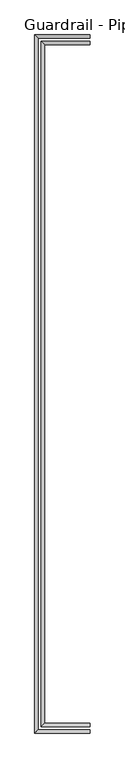
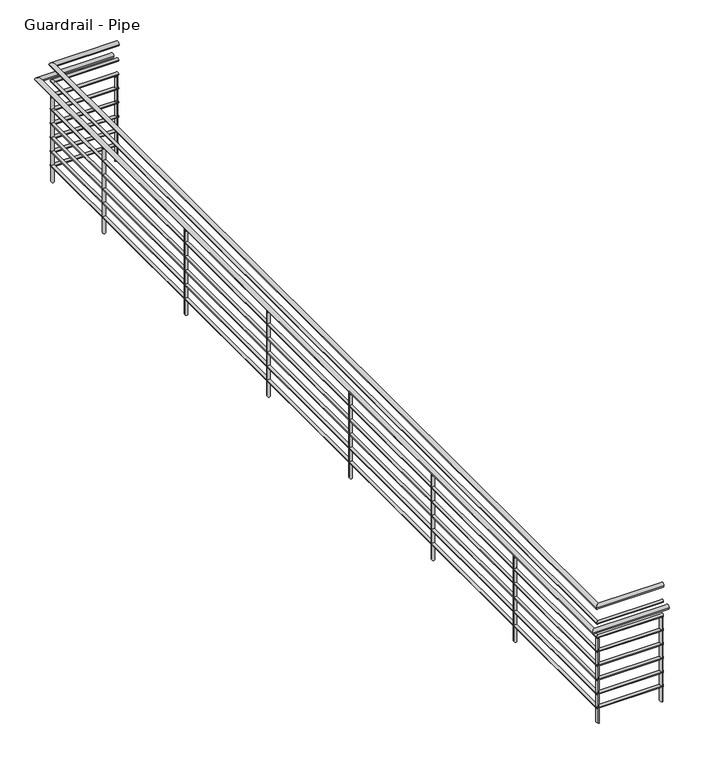
"""IFC4 building model written with IfcOpenShell, lengths in millimetres: railing geometry, Guardrail - Pipe."""

from ifc_helpers import new_model, si_unit, frame, origin, place, context, project, spatial, circle_curve, ellipse_curve, source, transform, mapped, element, save
from ifc_brep_helpers import plane_surface, cylinder_surface, advanced_brep


def guardrail_pipe_c5bc1630(model_context):
    return source(origin(), model_context, "Body", "AdvancedBrep", [
        advanced_brep(
        [(11534.3313551, 10867.95, 4705.35), (11534.3313551, 10906.05, 4705.35), (10956.4813551, 10867.95, 4705.35), (10994.5813551, 10906.05, 4705.35), (10956.4813551, 18983.25, 4705.35), (10994.5813551, 18945.15, 4705.35), (11534.3313551, 18983.25, 4705.35), (11534.3313551, 18945.15, 4705.35)],
        [
            (0, 1, circle_curve(frame((11534.3313551, 10887.0, 4705.35), z_axis=(1.0, 0.0, 0.0), x_axis=(0.0, 1.0, 0.0)), 19.05)),
            (1, 0, circle_curve(frame((11534.3313551, 10887.0, 4705.35), z_axis=(1.0, 0.0, 0.0), x_axis=(0.0, 1.0, 0.0)), 19.05)),
            (0, 2),
            (2, 3, ellipse_curve(frame((10975.5313551, 10887.0, 4705.35), z_axis=(0.7071067811865475, -0.7071067811865475, 0.0), x_axis=(0.7071067811865476, 0.7071067811865474, 0.0)), 26.9407684, 19.05)),
            (3, 1),
            (3, 2, ellipse_curve(frame((10975.5313551, 10887.0, 4705.35), z_axis=(0.7071067811865475, -0.7071067811865475, 0.0), x_axis=(0.7071067811865476, 0.7071067811865474, 0.0)), 26.9407684, 19.05)),
            (2, 4),
            (4, 5, ellipse_curve(frame((10975.5313551, 18964.2, 4705.35), z_axis=(-0.7071067811865475, -0.7071067811865475, 0.0), x_axis=(0.7071067811865474, -0.7071067811865476, 0.0)), 26.9407684, 19.05)),
            (5, 3),
            (5, 4, ellipse_curve(frame((10975.5313551, 18964.2, 4705.35), z_axis=(-0.7071067811865475, -0.7071067811865475, 0.0), x_axis=(0.7071067811865474, -0.7071067811865476, 0.0)), 26.9407684, 19.05)),
            (6, 7, circle_curve(frame((11534.3313551, 18964.2, 4705.35), z_axis=(1.0, 0.0, 0.0), x_axis=(0.0, -1.0, 0.0)), 19.05)),
            (7, 6, circle_curve(frame((11534.3313551, 18964.2, 4705.35), z_axis=(1.0, 0.0, 0.0), x_axis=(0.0, -1.0, 0.0)), 19.05)),
            (4, 6),
            (7, 5),
        ],
        [
            plane_surface(frame((11534.3313551, 10887.0, 4724.4), z_axis=(1.0, 0.0, 0.0), x_axis=(0.0, -1.0, 0.0))),
            cylinder_surface(frame((11534.3313551, 10887.0, 4705.35), z_axis=(1.0, 0.0, 0.0), x_axis=(0.0, 1.0, 0.0)), 19.05),
            cylinder_surface(frame((10975.5313551, 10887.0, 4705.35), z_axis=(0.0, -1.0, 0.0), x_axis=(1.0, 0.0, 0.0)), 19.05),
            plane_surface(frame((11534.3313551, 18964.2, 4724.4), z_axis=(1.0, 0.0, 0.0), x_axis=(0.0, 1.0, 0.0))),
            cylinder_surface(frame((10975.5313551, 18964.2, 4705.35), z_axis=(-1.0, 0.0, 0.0), x_axis=(0.0, -1.0, 0.0)), 19.05),
        ],
        [
            (0, [[1, 2]]),
            (1, [[-1, 3, 4, 5]]),
            (1, [[-2, -5, 6, -3]]),
            (2, [[-4, 7, 8, 9]]),
            (2, [[-6, -9, 10, -7]]),
            (3, [[11, 12]]),
            (4, [[-8, 13, -12, 14]]),
            (4, [[-10, -14, -11, -13]]),
        ],
    ),
        advanced_brep(
        [(11534.3313551, 10874.3, 4559.3), (11534.3313551, 10899.7, 4559.3), (10962.8313551, 10874.3, 4559.3), (10988.2313551, 10899.7, 4559.3), (10962.8313551, 18976.9, 4559.3), (10988.2313551, 18951.5, 4559.3), (11534.3313551, 18976.9, 4559.3), (11534.3313551, 18951.5, 4559.3)],
        [
            (0, 1, circle_curve(frame((11534.3313551, 10887.0, 4559.3), z_axis=(1.0, 0.0, 0.0), x_axis=(0.0, 1.0, 0.0)), 12.7)),
            (1, 0, circle_curve(frame((11534.3313551, 10887.0, 4559.3), z_axis=(1.0, 0.0, 0.0), x_axis=(0.0, 1.0, 0.0)), 12.7)),
            (0, 2),
            (2, 3, ellipse_curve(frame((10975.5313551, 10887.0, 4559.3), z_axis=(0.7071067811865475, -0.7071067811865475, 0.0), x_axis=(0.7071067811865476, 0.7071067811865474, 0.0)), 17.9605122, 12.7)),
            (3, 1),
            (3, 2, ellipse_curve(frame((10975.5313551, 10887.0, 4559.3), z_axis=(0.7071067811865475, -0.7071067811865475, 0.0), x_axis=(0.7071067811865476, 0.7071067811865474, 0.0)), 17.9605122, 12.7)),
            (2, 4),
            (4, 5, ellipse_curve(frame((10975.5313551, 18964.2, 4559.3), z_axis=(-0.7071067811865475, -0.7071067811865475, 0.0), x_axis=(0.7071067811865474, -0.7071067811865476, 0.0)), 17.9605122, 12.7)),
            (5, 3),
            (5, 4, ellipse_curve(frame((10975.5313551, 18964.2, 4559.3), z_axis=(-0.7071067811865475, -0.7071067811865475, 0.0), x_axis=(0.7071067811865474, -0.7071067811865476, 0.0)), 17.9605122, 12.7)),
            (6, 7, circle_curve(frame((11534.3313551, 18964.2, 4559.3), z_axis=(1.0, 0.0, 0.0), x_axis=(0.0, -1.0, 0.0)), 12.7)),
            (7, 6, circle_curve(frame((11534.3313551, 18964.2, 4559.3), z_axis=(1.0, 0.0, 0.0), x_axis=(0.0, -1.0, 0.0)), 12.7)),
            (4, 6),
            (7, 5),
        ],
        [
            plane_surface(frame((11534.3313551, 10887.0, 4572.0), z_axis=(1.0, 0.0, 0.0), x_axis=(0.0, -1.0, 0.0))),
            cylinder_surface(frame((11534.3313551, 10887.0, 4559.3), z_axis=(1.0, 0.0, 0.0), x_axis=(0.0, 1.0, 0.0)), 12.7),
            cylinder_surface(frame((10975.5313551, 10887.0, 4559.3), z_axis=(0.0, -1.0, 0.0), x_axis=(1.0, 0.0, 0.0)), 12.7),
            plane_surface(frame((11534.3313551, 18964.2, 4572.0), z_axis=(1.0, 0.0, 0.0), x_axis=(0.0, 1.0, 0.0))),
            cylinder_surface(frame((10975.5313551, 18964.2, 4559.3), z_axis=(-1.0, 0.0, 0.0), x_axis=(0.0, -1.0, 0.0)), 12.7),
        ],
        [
            (0, [[1, 2]]),
            (1, [[-1, 3, 4, 5]]),
            (1, [[-2, -5, 6, -3]]),
            (2, [[-4, 7, 8, 9]]),
            (2, [[-6, -9, 10, -7]]),
            (3, [[11, 12]]),
            (4, [[-8, 13, -12, 14]]),
            (4, [[-10, -14, -11, -13]]),
        ],
    ),
        advanced_brep(
        [(11534.3313551, 10791.75, 4552.95), (11534.3313551, 10829.85, 4552.95), (10880.2813551, 10791.75, 4552.95), (10918.3813551, 10829.85, 4552.95), (10880.2813551, 19059.45, 4552.95), (10918.3813551, 19021.35, 4552.95), (11534.3313551, 19059.45, 4552.95), (11534.3313551, 19021.35, 4552.95)],
        [
            (0, 1, circle_curve(frame((11534.3313551, 10810.8, 4552.95), z_axis=(1.0, 0.0, 0.0), x_axis=(0.0, 1.0, 0.0)), 19.05)),
            (1, 0, circle_curve(frame((11534.3313551, 10810.8, 4552.95), z_axis=(1.0, 0.0, 0.0), x_axis=(0.0, 1.0, 0.0)), 19.05)),
            (0, 2),
            (2, 3, ellipse_curve(frame((10899.3313551, 10810.8, 4552.95), z_axis=(0.7071067811865475, -0.7071067811865475, 0.0), x_axis=(0.7071067811865476, 0.7071067811865474, 0.0)), 26.9407684, 19.05)),
            (3, 1),
            (3, 2, ellipse_curve(frame((10899.3313551, 10810.8, 4552.95), z_axis=(0.7071067811865475, -0.7071067811865475, 0.0), x_axis=(0.7071067811865476, 0.7071067811865474, 0.0)), 26.9407684, 19.05)),
            (2, 4),
            (4, 5, ellipse_curve(frame((10899.3313551, 19040.4, 4552.95), z_axis=(-0.7071067811865475, -0.7071067811865475, 0.0), x_axis=(0.7071067811865474, -0.7071067811865476, 0.0)), 26.9407684, 19.05)),
            (5, 3),
            (5, 4, ellipse_curve(frame((10899.3313551, 19040.4, 4552.95), z_axis=(-0.7071067811865475, -0.7071067811865475, 0.0), x_axis=(0.7071067811865474, -0.7071067811865476, 0.0)), 26.9407684, 19.05)),
            (6, 7, circle_curve(frame((11534.3313551, 19040.4, 4552.95), z_axis=(1.0, 0.0, 0.0), x_axis=(0.0, -1.0, 0.0)), 19.05)),
            (7, 6, circle_curve(frame((11534.3313551, 19040.4, 4552.95), z_axis=(1.0, 0.0, 0.0), x_axis=(0.0, -1.0, 0.0)), 19.05)),
            (4, 6),
            (7, 5),
        ],
        [
            plane_surface(frame((11534.3313551, 10810.8, 4572.0), z_axis=(1.0, 0.0, 0.0), x_axis=(0.0, -1.0, 0.0))),
            cylinder_surface(frame((11534.3313551, 10810.8, 4552.95), z_axis=(1.0, 0.0, 0.0), x_axis=(0.0, 1.0, 0.0)), 19.05),
            cylinder_surface(frame((10899.3313551, 10810.8, 4552.95), z_axis=(0.0, -1.0, 0.0), x_axis=(1.0, 0.0, 0.0)), 19.05),
            plane_surface(frame((11534.3313551, 19040.4, 4572.0), z_axis=(1.0, 0.0, 0.0), x_axis=(0.0, 1.0, 0.0))),
            cylinder_surface(frame((10899.3313551, 19040.4, 4552.95), z_axis=(-1.0, 0.0, 0.0), x_axis=(0.0, -1.0, 0.0)), 19.05),
        ],
        [
            (0, [[1, 2]]),
            (1, [[-1, 3, 4, 5]]),
            (1, [[-2, -5, 6, -3]]),
            (2, [[-4, 7, 8, 9]]),
            (2, [[-6, -9, 10, -7]]),
            (3, [[11, 12]]),
            (4, [[-8, 13, -12, 14]]),
            (4, [[-10, -14, -11, -13]]),
        ],
    ),
        advanced_brep(
        [(11534.3313551, 10874.3, 4432.3), (11534.3313551, 10899.7, 4432.3), (10962.8313551, 10874.3, 4432.3), (10988.2313551, 10899.7, 4432.3), (10962.8313551, 18976.9, 4432.3), (10988.2313551, 18951.5, 4432.3), (11534.3313551, 18976.9, 4432.3), (11534.3313551, 18951.5, 4432.3)],
        [
            (0, 1, circle_curve(frame((11534.3313551, 10887.0, 4432.3), z_axis=(1.0, 0.0, 0.0), x_axis=(0.0, 1.0, 0.0)), 12.7)),
            (1, 0, circle_curve(frame((11534.3313551, 10887.0, 4432.3), z_axis=(1.0, 0.0, 0.0), x_axis=(0.0, 1.0, 0.0)), 12.7)),
            (0, 2),
            (2, 3, ellipse_curve(frame((10975.5313551, 10887.0, 4432.3), z_axis=(0.7071067811865475, -0.7071067811865475, 0.0), x_axis=(0.7071067811865476, 0.7071067811865474, 0.0)), 17.9605122, 12.7)),
            (3, 1),
            (3, 2, ellipse_curve(frame((10975.5313551, 10887.0, 4432.3), z_axis=(0.7071067811865475, -0.7071067811865475, 0.0), x_axis=(0.7071067811865476, 0.7071067811865474, 0.0)), 17.9605122, 12.7)),
            (2, 4),
            (4, 5, ellipse_curve(frame((10975.5313551, 18964.2, 4432.3), z_axis=(-0.7071067811865475, -0.7071067811865475, 0.0), x_axis=(0.7071067811865474, -0.7071067811865476, 0.0)), 17.9605122, 12.7)),
            (5, 3),
            (5, 4, ellipse_curve(frame((10975.5313551, 18964.2, 4432.3), z_axis=(-0.7071067811865475, -0.7071067811865475, 0.0), x_axis=(0.7071067811865474, -0.7071067811865476, 0.0)), 17.9605122, 12.7)),
            (6, 7, circle_curve(frame((11534.3313551, 18964.2, 4432.3), z_axis=(1.0, 0.0, 0.0), x_axis=(0.0, -1.0, 0.0)), 12.7)),
            (7, 6, circle_curve(frame((11534.3313551, 18964.2, 4432.3), z_axis=(1.0, 0.0, 0.0), x_axis=(0.0, -1.0, 0.0)), 12.7)),
            (4, 6),
            (7, 5),
        ],
        [
            plane_surface(frame((11534.3313551, 10887.0, 4445.0), z_axis=(1.0, 0.0, 0.0), x_axis=(0.0, -1.0, 0.0))),
            cylinder_surface(frame((11534.3313551, 10887.0, 4432.3), z_axis=(1.0, 0.0, 0.0), x_axis=(0.0, 1.0, 0.0)), 12.7),
            cylinder_surface(frame((10975.5313551, 10887.0, 4432.3), z_axis=(0.0, -1.0, 0.0), x_axis=(1.0, 0.0, 0.0)), 12.7),
            plane_surface(frame((11534.3313551, 18964.2, 4445.0), z_axis=(1.0, 0.0, 0.0), x_axis=(0.0, 1.0, 0.0))),
            cylinder_surface(frame((10975.5313551, 18964.2, 4432.3), z_axis=(-1.0, 0.0, 0.0), x_axis=(0.0, -1.0, 0.0)), 12.7),
        ],
        [
            (0, [[1, 2]]),
            (1, [[-1, 3, 4, 5]]),
            (1, [[-2, -5, 6, -3]]),
            (2, [[-4, 7, 8, 9]]),
            (2, [[-6, -9, 10, -7]]),
            (3, [[11, 12]]),
            (4, [[-8, 13, -12, 14]]),
            (4, [[-10, -14, -11, -13]]),
        ],
    ),
        advanced_brep(
        [(11534.3313551, 10874.3, 4305.3), (11534.3313551, 10899.7, 4305.3), (10962.8313551, 10874.3, 4305.3), (10988.2313551, 10899.7, 4305.3), (10962.8313551, 18976.9, 4305.3), (10988.2313551, 18951.5, 4305.3), (11534.3313551, 18976.9, 4305.3), (11534.3313551, 18951.5, 4305.3)],
        [
            (0, 1, circle_curve(frame((11534.3313551, 10887.0, 4305.3), z_axis=(1.0, 0.0, 0.0), x_axis=(0.0, 1.0, 0.0)), 12.7)),
            (1, 0, circle_curve(frame((11534.3313551, 10887.0, 4305.3), z_axis=(1.0, 0.0, 0.0), x_axis=(0.0, 1.0, 0.0)), 12.7)),
            (0, 2),
            (2, 3, ellipse_curve(frame((10975.5313551, 10887.0, 4305.3), z_axis=(0.7071067811865475, -0.7071067811865475, 0.0), x_axis=(0.7071067811865476, 0.7071067811865474, 0.0)), 17.9605122, 12.7)),
            (3, 1),
            (3, 2, ellipse_curve(frame((10975.5313551, 10887.0, 4305.3), z_axis=(0.7071067811865475, -0.7071067811865475, 0.0), x_axis=(0.7071067811865476, 0.7071067811865474, 0.0)), 17.9605122, 12.7)),
            (2, 4),
            (4, 5, ellipse_curve(frame((10975.5313551, 18964.2, 4305.3), z_axis=(-0.7071067811865475, -0.7071067811865475, 0.0), x_axis=(0.7071067811865474, -0.7071067811865476, 0.0)), 17.9605122, 12.7)),
            (5, 3),
            (5, 4, ellipse_curve(frame((10975.5313551, 18964.2, 4305.3), z_axis=(-0.7071067811865475, -0.7071067811865475, 0.0), x_axis=(0.7071067811865474, -0.7071067811865476, 0.0)), 17.9605122, 12.7)),
            (6, 7, circle_curve(frame((11534.3313551, 18964.2, 4305.3), z_axis=(1.0, 0.0, 0.0), x_axis=(0.0, -1.0, 0.0)), 12.7)),
            (7, 6, circle_curve(frame((11534.3313551, 18964.2, 4305.3), z_axis=(1.0, 0.0, 0.0), x_axis=(0.0, -1.0, 0.0)), 12.7)),
            (4, 6),
            (7, 5),
        ],
        [
            plane_surface(frame((11534.3313551, 10887.0, 4318.0), z_axis=(1.0, 0.0, 0.0), x_axis=(0.0, -1.0, 0.0))),
            cylinder_surface(frame((11534.3313551, 10887.0, 4305.3), z_axis=(1.0, 0.0, 0.0), x_axis=(0.0, 1.0, 0.0)), 12.7),
            cylinder_surface(frame((10975.5313551, 10887.0, 4305.3), z_axis=(0.0, -1.0, 0.0), x_axis=(1.0, 0.0, 0.0)), 12.7),
            plane_surface(frame((11534.3313551, 18964.2, 4318.0), z_axis=(1.0, 0.0, 0.0), x_axis=(0.0, 1.0, 0.0))),
            cylinder_surface(frame((10975.5313551, 18964.2, 4305.3), z_axis=(-1.0, 0.0, 0.0), x_axis=(0.0, -1.0, 0.0)), 12.7),
        ],
        [
            (0, [[1, 2]]),
            (1, [[-1, 3, 4, 5]]),
            (1, [[-2, -5, 6, -3]]),
            (2, [[-4, 7, 8, 9]]),
            (2, [[-6, -9, 10, -7]]),
            (3, [[11, 12]]),
            (4, [[-8, 13, -12, 14]]),
            (4, [[-10, -14, -11, -13]]),
        ],
    ),
        advanced_brep(
        [(11534.3313551, 10874.3, 4178.3), (11534.3313551, 10899.7, 4178.3), (10962.8313551, 10874.3, 4178.3), (10988.2313551, 10899.7, 4178.3), (10962.8313551, 18976.9, 4178.3), (10988.2313551, 18951.5, 4178.3), (11534.3313551, 18976.9, 4178.3), (11534.3313551, 18951.5, 4178.3)],
        [
            (0, 1, circle_curve(frame((11534.3313551, 10887.0, 4178.3), z_axis=(1.0, 0.0, 0.0), x_axis=(0.0, 1.0, 0.0)), 12.7)),
            (1, 0, circle_curve(frame((11534.3313551, 10887.0, 4178.3), z_axis=(1.0, 0.0, 0.0), x_axis=(0.0, 1.0, 0.0)), 12.7)),
            (0, 2),
            (2, 3, ellipse_curve(frame((10975.5313551, 10887.0, 4178.3), z_axis=(0.7071067811865475, -0.7071067811865475, 0.0), x_axis=(0.7071067811865476, 0.7071067811865474, 0.0)), 17.9605122, 12.7)),
            (3, 1),
            (3, 2, ellipse_curve(frame((10975.5313551, 10887.0, 4178.3), z_axis=(0.7071067811865475, -0.7071067811865475, 0.0), x_axis=(0.7071067811865476, 0.7071067811865474, 0.0)), 17.9605122, 12.7)),
            (2, 4),
            (4, 5, ellipse_curve(frame((10975.5313551, 18964.2, 4178.3), z_axis=(-0.7071067811865475, -0.7071067811865475, 0.0), x_axis=(0.7071067811865474, -0.7071067811865476, 0.0)), 17.9605122, 12.7)),
            (5, 3),
            (5, 4, ellipse_curve(frame((10975.5313551, 18964.2, 4178.3), z_axis=(-0.7071067811865475, -0.7071067811865475, 0.0), x_axis=(0.7071067811865474, -0.7071067811865476, 0.0)), 17.9605122, 12.7)),
            (6, 7, circle_curve(frame((11534.3313551, 18964.2, 4178.3), z_axis=(1.0, 0.0, 0.0), x_axis=(0.0, -1.0, 0.0)), 12.7)),
            (7, 6, circle_curve(frame((11534.3313551, 18964.2, 4178.3), z_axis=(1.0, 0.0, 0.0), x_axis=(0.0, -1.0, 0.0)), 12.7)),
            (4, 6),
            (7, 5),
        ],
        [
            plane_surface(frame((11534.3313551, 10887.0, 4191.0), z_axis=(1.0, 0.0, 0.0), x_axis=(0.0, -1.0, 0.0))),
            cylinder_surface(frame((11534.3313551, 10887.0, 4178.3), z_axis=(1.0, 0.0, 0.0), x_axis=(0.0, 1.0, 0.0)), 12.7),
            cylinder_surface(frame((10975.5313551, 10887.0, 4178.3), z_axis=(0.0, -1.0, 0.0), x_axis=(1.0, 0.0, 0.0)), 12.7),
            plane_surface(frame((11534.3313551, 18964.2, 4191.0), z_axis=(1.0, 0.0, 0.0), x_axis=(0.0, 1.0, 0.0))),
            cylinder_surface(frame((10975.5313551, 18964.2, 4178.3), z_axis=(-1.0, 0.0, 0.0), x_axis=(0.0, -1.0, 0.0)), 12.7),
        ],
        [
            (0, [[1, 2]]),
            (1, [[-1, 3, 4, 5]]),
            (1, [[-2, -5, 6, -3]]),
            (2, [[-4, 7, 8, 9]]),
            (2, [[-6, -9, 10, -7]]),
            (3, [[11, 12]]),
            (4, [[-8, 13, -12, 14]]),
            (4, [[-10, -14, -11, -13]]),
        ],
    ),
        advanced_brep(
        [(11534.3313551, 10874.3, 4051.3), (11534.3313551, 10899.7, 4051.3), (10962.8313551, 10874.3, 4051.3), (10988.2313551, 10899.7, 4051.3), (10962.8313551, 18976.9, 4051.3), (10988.2313551, 18951.5, 4051.3), (11534.3313551, 18976.9, 4051.3), (11534.3313551, 18951.5, 4051.3)],
        [
            (0, 1, circle_curve(frame((11534.3313551, 10887.0, 4051.3), z_axis=(1.0, 0.0, 0.0), x_axis=(0.0, 1.0, 0.0)), 12.7)),
            (1, 0, circle_curve(frame((11534.3313551, 10887.0, 4051.3), z_axis=(1.0, 0.0, 0.0), x_axis=(0.0, 1.0, 0.0)), 12.7)),
            (0, 2),
            (2, 3, ellipse_curve(frame((10975.5313551, 10887.0, 4051.3), z_axis=(0.7071067811865475, -0.7071067811865475, 0.0), x_axis=(0.7071067811865476, 0.7071067811865474, 0.0)), 17.9605122, 12.7)),
            (3, 1),
            (3, 2, ellipse_curve(frame((10975.5313551, 10887.0, 4051.3), z_axis=(0.7071067811865475, -0.7071067811865475, 0.0), x_axis=(0.7071067811865476, 0.7071067811865474, 0.0)), 17.9605122, 12.7)),
            (2, 4),
            (4, 5, ellipse_curve(frame((10975.5313551, 18964.2, 4051.3), z_axis=(-0.7071067811865475, -0.7071067811865475, 0.0), x_axis=(0.7071067811865474, -0.7071067811865476, 0.0)), 17.9605122, 12.7)),
            (5, 3),
            (5, 4, ellipse_curve(frame((10975.5313551, 18964.2, 4051.3), z_axis=(-0.7071067811865475, -0.7071067811865475, 0.0), x_axis=(0.7071067811865474, -0.7071067811865476, 0.0)), 17.9605122, 12.7)),
            (6, 7, circle_curve(frame((11534.3313551, 18964.2, 4051.3), z_axis=(1.0, 0.0, 0.0), x_axis=(0.0, -1.0, 0.0)), 12.7)),
            (7, 6, circle_curve(frame((11534.3313551, 18964.2, 4051.3), z_axis=(1.0, 0.0, 0.0), x_axis=(0.0, -1.0, 0.0)), 12.7)),
            (4, 6),
            (7, 5),
        ],
        [
            plane_surface(frame((11534.3313551, 10887.0, 4064.0), z_axis=(1.0, 0.0, 0.0), x_axis=(0.0, -1.0, 0.0))),
            cylinder_surface(frame((11534.3313551, 10887.0, 4051.3), z_axis=(1.0, 0.0, 0.0), x_axis=(0.0, 1.0, 0.0)), 12.7),
            cylinder_surface(frame((10975.5313551, 10887.0, 4051.3), z_axis=(0.0, -1.0, 0.0), x_axis=(1.0, 0.0, 0.0)), 12.7),
            plane_surface(frame((11534.3313551, 18964.2, 4064.0), z_axis=(1.0, 0.0, 0.0), x_axis=(0.0, 1.0, 0.0))),
            cylinder_surface(frame((10975.5313551, 18964.2, 4051.3), z_axis=(-1.0, 0.0, 0.0), x_axis=(0.0, -1.0, 0.0)), 12.7),
        ],
        [
            (0, [[1, 2]]),
            (1, [[-1, 3, 4, 5]]),
            (1, [[-2, -5, 6, -3]]),
            (2, [[-4, 7, 8, 9]]),
            (2, [[-6, -9, 10, -7]]),
            (3, [[11, 12]]),
            (4, [[-8, 13, -12, 14]]),
            (4, [[-10, -14, -11, -13]]),
        ],
    ),
        advanced_brep(
        [(11534.3313551, 10874.3, 3924.3), (11534.3313551, 10899.7, 3924.3), (10962.8313551, 10874.3, 3924.3), (10988.2313551, 10899.7, 3924.3), (10962.8313551, 18976.9, 3924.3), (10988.2313551, 18951.5, 3924.3), (11534.3313551, 18976.9, 3924.3), (11534.3313551, 18951.5, 3924.3)],
        [
            (0, 1, circle_curve(frame((11534.3313551, 10887.0, 3924.3), z_axis=(1.0, 0.0, 0.0), x_axis=(0.0, 1.0, 0.0)), 12.7)),
            (1, 0, circle_curve(frame((11534.3313551, 10887.0, 3924.3), z_axis=(1.0, 0.0, 0.0), x_axis=(0.0, 1.0, 0.0)), 12.7)),
            (0, 2),
            (2, 3, ellipse_curve(frame((10975.5313551, 10887.0, 3924.3), z_axis=(0.7071067811865475, -0.7071067811865475, 0.0), x_axis=(0.7071067811865476, 0.7071067811865474, 0.0)), 17.9605122, 12.7)),
            (3, 1),
            (3, 2, ellipse_curve(frame((10975.5313551, 10887.0, 3924.3), z_axis=(0.7071067811865475, -0.7071067811865475, 0.0), x_axis=(0.7071067811865476, 0.7071067811865474, 0.0)), 17.9605122, 12.7)),
            (2, 4),
            (4, 5, ellipse_curve(frame((10975.5313551, 18964.2, 3924.3), z_axis=(-0.7071067811865475, -0.7071067811865475, 0.0), x_axis=(0.7071067811865474, -0.7071067811865476, 0.0)), 17.9605122, 12.7)),
            (5, 3),
            (5, 4, ellipse_curve(frame((10975.5313551, 18964.2, 3924.3), z_axis=(-0.7071067811865475, -0.7071067811865475, 0.0), x_axis=(0.7071067811865474, -0.7071067811865476, 0.0)), 17.9605122, 12.7)),
            (6, 7, circle_curve(frame((11534.3313551, 18964.2, 3924.3), z_axis=(1.0, 0.0, 0.0), x_axis=(0.0, -1.0, 0.0)), 12.7)),
            (7, 6, circle_curve(frame((11534.3313551, 18964.2, 3924.3), z_axis=(1.0, 0.0, 0.0), x_axis=(0.0, -1.0, 0.0)), 12.7)),
            (4, 6),
            (7, 5),
        ],
        [
            plane_surface(frame((11534.3313551, 10887.0, 3937.0), z_axis=(1.0, 0.0, 0.0), x_axis=(0.0, -1.0, 0.0))),
            cylinder_surface(frame((11534.3313551, 10887.0, 3924.3), z_axis=(1.0, 0.0, 0.0), x_axis=(0.0, 1.0, 0.0)), 12.7),
            cylinder_surface(frame((10975.5313551, 10887.0, 3924.3), z_axis=(0.0, -1.0, 0.0), x_axis=(1.0, 0.0, 0.0)), 12.7),
            plane_surface(frame((11534.3313551, 18964.2, 3937.0), z_axis=(1.0, 0.0, 0.0), x_axis=(0.0, 1.0, 0.0))),
            cylinder_surface(frame((10975.5313551, 18964.2, 3924.3), z_axis=(-1.0, 0.0, 0.0), x_axis=(0.0, -1.0, 0.0)), 12.7),
        ],
        [
            (0, [[1, 2]]),
            (1, [[-1, 3, 4, 5]]),
            (1, [[-2, -5, 6, -3]]),
            (2, [[-4, 7, 8, 9]]),
            (2, [[-6, -9, 10, -7]]),
            (3, [[11, 12]]),
            (4, [[-8, 13, -12, 14]]),
            (4, [[-10, -14, -11, -13]]),
        ],
    ),
        advanced_brep(
        [(11534.3313551, 10874.3, 3797.3), (11534.3313551, 10899.7, 3797.3), (10962.8313551, 10874.3, 3797.3), (10988.2313551, 10899.7, 3797.3), (10962.8313551, 18976.9, 3797.3), (10988.2313551, 18951.5, 3797.3), (11534.3313551, 18976.9, 3797.3), (11534.3313551, 18951.5, 3797.3)],
        [
            (0, 1, circle_curve(frame((11534.3313551, 10887.0, 3797.3), z_axis=(1.0, 0.0, 0.0), x_axis=(0.0, 1.0, 0.0)), 12.7)),
            (1, 0, circle_curve(frame((11534.3313551, 10887.0, 3797.3), z_axis=(1.0, 0.0, 0.0), x_axis=(0.0, 1.0, 0.0)), 12.7)),
            (0, 2),
            (2, 3, ellipse_curve(frame((10975.5313551, 10887.0, 3797.3), z_axis=(0.7071067811865475, -0.7071067811865475, 0.0), x_axis=(0.7071067811865476, 0.7071067811865474, 0.0)), 17.9605122, 12.7)),
            (3, 1),
            (3, 2, ellipse_curve(frame((10975.5313551, 10887.0, 3797.3), z_axis=(0.7071067811865475, -0.7071067811865475, 0.0), x_axis=(0.7071067811865476, 0.7071067811865474, 0.0)), 17.9605122, 12.7)),
            (2, 4),
            (4, 5, ellipse_curve(frame((10975.5313551, 18964.2, 3797.3), z_axis=(-0.7071067811865475, -0.7071067811865475, 0.0), x_axis=(0.7071067811865474, -0.7071067811865476, 0.0)), 17.9605122, 12.7)),
            (5, 3),
            (5, 4, ellipse_curve(frame((10975.5313551, 18964.2, 3797.3), z_axis=(-0.7071067811865475, -0.7071067811865475, 0.0), x_axis=(0.7071067811865474, -0.7071067811865476, 0.0)), 17.9605122, 12.7)),
            (6, 7, circle_curve(frame((11534.3313551, 18964.2, 3797.3), z_axis=(1.0, 0.0, 0.0), x_axis=(0.0, -1.0, 0.0)), 12.7)),
            (7, 6, circle_curve(frame((11534.3313551, 18964.2, 3797.3), z_axis=(1.0, 0.0, 0.0), x_axis=(0.0, -1.0, 0.0)), 12.7)),
            (4, 6),
            (7, 5),
        ],
        [
            plane_surface(frame((11534.3313551, 10887.0, 3810.0), z_axis=(1.0, 0.0, 0.0), x_axis=(0.0, -1.0, 0.0))),
            cylinder_surface(frame((11534.3313551, 10887.0, 3797.3), z_axis=(1.0, 0.0, 0.0), x_axis=(0.0, 1.0, 0.0)), 12.7),
            cylinder_surface(frame((10975.5313551, 10887.0, 3797.3), z_axis=(0.0, -1.0, 0.0), x_axis=(1.0, 0.0, 0.0)), 12.7),
            plane_surface(frame((11534.3313551, 18964.2, 3810.0), z_axis=(1.0, 0.0, 0.0), x_axis=(0.0, 1.0, 0.0))),
            cylinder_surface(frame((10975.5313551, 18964.2, 3797.3), z_axis=(-1.0, 0.0, 0.0), x_axis=(0.0, -1.0, 0.0)), 12.7),
        ],
        [
            (0, [[1, 2]]),
            (1, [[-1, 3, 4, 5]]),
            (1, [[-2, -5, 6, -3]]),
            (2, [[-4, 7, 8, 9]]),
            (2, [[-6, -9, 10, -7]]),
            (3, [[11, 12]]),
            (4, [[-8, 13, -12, 14]]),
            (4, [[-10, -14, -11, -13]]),
        ],
    ),
        advanced_brep(
        [(10988.2313551, 18202.2, 4419.6), (10988.2313551, 18202.2, 3657.6), (10962.8313551, 18202.2, 3657.6), (10962.8313551, 18202.2, 4419.6)],
        [
            (0, 1),
            (1, 2, ellipse_curve(frame((10975.5313551, 18202.2, 3657.6), z_axis=(0.0, -0.536857935986758, 0.8436726596068158), x_axis=(0.0, 0.8436726596068159, 0.536857935986758)), 15.0532317, 12.7)),
            (2, 3),
            (3, 0, ellipse_curve(frame((10975.5313551, 18202.2, 4419.6), z_axis=(0.0, 0.5368579359867546, -0.8436726596068179), x_axis=(0.0, 0.843672659606818, 0.5368579359867547)), 15.0532317, 12.7)),
            (0, 3, ellipse_curve(frame((10975.5313551, 18202.2, 4419.6), z_axis=(0.0, 0.5368579359867546, -0.8436726596068179), x_axis=(0.0, 0.843672659606818, 0.5368579359867547)), 15.0532317, 12.7)),
            (2, 1, ellipse_curve(frame((10975.5313551, 18202.2, 3657.6), z_axis=(0.0, -0.536857935986758, 0.8436726596068158), x_axis=(0.0, 0.8436726596068159, 0.536857935986758)), 15.0532317, 12.7)),
        ],
        [
            cylinder_surface(frame((10975.5313551, 18202.2, 3429.0), z_axis=(0.0, 0.0, 1.0), x_axis=(-1.0, 0.0, 0.0)), 12.7),
            plane_surface(frame((10950.1313551, 18227.6, 4435.7628938), z_axis=(0.0, -0.5368579359867546, 0.8436726596068179), x_axis=(1.0, 0.0, 0.0))),
            plane_surface(frame((10950.1313551, 18176.8, 3641.4371062), z_axis=(0.0, 0.536857935986758, -0.8436726596068158), x_axis=(1.0, 0.0, 0.0))),
        ],
        [
            (0, [[1, 2, 3, 4]]),
            (0, [[-1, 5, -3, 6]]),
            (1, [[-4, -5]]),
            (2, [[-2, -6]]),
        ],
    ),
        advanced_brep(
        [(10988.2313551, 16983.0, 4419.6), (10988.2313551, 16983.0, 3657.6), (10962.8313551, 16983.0, 3657.6), (10962.8313551, 16983.0, 4419.6)],
        [
            (0, 1),
            (1, 2, ellipse_curve(frame((10975.5313551, 16983.0, 3657.6), z_axis=(0.0, -0.536857935986758, 0.8436726596068158), x_axis=(0.0, 0.8436726596068159, 0.536857935986758)), 15.0532317, 12.7)),
            (2, 3),
            (3, 0, ellipse_curve(frame((10975.5313551, 16983.0, 4419.6), z_axis=(0.0, 0.5368579359867546, -0.8436726596068179), x_axis=(0.0, 0.843672659606818, 0.5368579359867547)), 15.0532317, 12.7)),
            (0, 3, ellipse_curve(frame((10975.5313551, 16983.0, 4419.6), z_axis=(0.0, 0.5368579359867546, -0.8436726596068179), x_axis=(0.0, 0.843672659606818, 0.5368579359867547)), 15.0532317, 12.7)),
            (2, 1, ellipse_curve(frame((10975.5313551, 16983.0, 3657.6), z_axis=(0.0, -0.536857935986758, 0.8436726596068158), x_axis=(0.0, 0.8436726596068159, 0.536857935986758)), 15.0532317, 12.7)),
        ],
        [
            cylinder_surface(frame((10975.5313551, 16983.0, 3429.0), z_axis=(0.0, 0.0, 1.0), x_axis=(-1.0, 0.0, 0.0)), 12.7),
            plane_surface(frame((10950.1313551, 17008.4, 4435.7628938), z_axis=(0.0, -0.5368579359867546, 0.8436726596068179), x_axis=(1.0, 0.0, 0.0))),
            plane_surface(frame((10950.1313551, 16957.6, 3641.4371062), z_axis=(0.0, 0.536857935986758, -0.8436726596068158), x_axis=(1.0, 0.0, 0.0))),
        ],
        [
            (0, [[1, 2, 3, 4]]),
            (0, [[-1, 5, -3, 6]]),
            (1, [[-4, -5]]),
            (2, [[-2, -6]]),
        ],
    ),
        advanced_brep(
        [(10988.2313551, 15763.8, 4419.6), (10988.2313551, 15763.8, 3657.6), (10962.8313551, 15763.8, 3657.6), (10962.8313551, 15763.8, 4419.6)],
        [
            (0, 1),
            (1, 2, ellipse_curve(frame((10975.5313551, 15763.8, 3657.6), z_axis=(0.0, -0.536857935986758, 0.8436726596068158), x_axis=(0.0, 0.8436726596068159, 0.536857935986758)), 15.0532317, 12.7)),
            (2, 3),
            (3, 0, ellipse_curve(frame((10975.5313551, 15763.8, 4419.6), z_axis=(0.0, 0.5368579359867546, -0.8436726596068179), x_axis=(0.0, 0.843672659606818, 0.5368579359867547)), 15.0532317, 12.7)),
            (0, 3, ellipse_curve(frame((10975.5313551, 15763.8, 4419.6), z_axis=(0.0, 0.5368579359867546, -0.8436726596068179), x_axis=(0.0, 0.843672659606818, 0.5368579359867547)), 15.0532317, 12.7)),
            (2, 1, ellipse_curve(frame((10975.5313551, 15763.8, 3657.6), z_axis=(0.0, -0.536857935986758, 0.8436726596068158), x_axis=(0.0, 0.8436726596068159, 0.536857935986758)), 15.0532317, 12.7)),
        ],
        [
            cylinder_surface(frame((10975.5313551, 15763.8, 3429.0), z_axis=(0.0, 0.0, 1.0), x_axis=(-1.0, 0.0, 0.0)), 12.7),
            plane_surface(frame((10950.1313551, 15789.2, 4435.7628938), z_axis=(0.0, -0.5368579359867546, 0.8436726596068179), x_axis=(1.0, 0.0, 0.0))),
            plane_surface(frame((10950.1313551, 15738.4, 3641.4371062), z_axis=(0.0, 0.536857935986758, -0.8436726596068158), x_axis=(1.0, 0.0, 0.0))),
        ],
        [
            (0, [[1, 2, 3, 4]]),
            (0, [[-1, 5, -3, 6]]),
            (1, [[-4, -5]]),
            (2, [[-2, -6]]),
        ],
    ),
        advanced_brep(
        [(10988.2313551, 14544.6, 4419.6), (10988.2313551, 14544.6, 3657.6), (10962.8313551, 14544.6, 3657.6), (10962.8313551, 14544.6, 4419.6)],
        [
            (0, 1),
            (1, 2, ellipse_curve(frame((10975.5313551, 14544.6, 3657.6), z_axis=(0.0, -0.536857935986758, 0.8436726596068158), x_axis=(0.0, 0.8436726596068159, 0.536857935986758)), 15.0532317, 12.7)),
            (2, 3),
            (3, 0, ellipse_curve(frame((10975.5313551, 14544.6, 4419.6), z_axis=(0.0, 0.5368579359867546, -0.8436726596068179), x_axis=(0.0, 0.843672659606818, 0.5368579359867547)), 15.0532317, 12.7)),
            (0, 3, ellipse_curve(frame((10975.5313551, 14544.6, 4419.6), z_axis=(0.0, 0.5368579359867546, -0.8436726596068179), x_axis=(0.0, 0.843672659606818, 0.5368579359867547)), 15.0532317, 12.7)),
            (2, 1, ellipse_curve(frame((10975.5313551, 14544.6, 3657.6), z_axis=(0.0, -0.536857935986758, 0.8436726596068158), x_axis=(0.0, 0.8436726596068159, 0.536857935986758)), 15.0532317, 12.7)),
        ],
        [
            cylinder_surface(frame((10975.5313551, 14544.6, 3429.0), z_axis=(0.0, 0.0, 1.0), x_axis=(-1.0, 0.0, 0.0)), 12.7),
            plane_surface(frame((10950.1313551, 14570.0, 4435.7628938), z_axis=(0.0, -0.5368579359867546, 0.8436726596068179), x_axis=(1.0, 0.0, 0.0))),
            plane_surface(frame((10950.1313551, 14519.2, 3641.4371062), z_axis=(0.0, 0.536857935986758, -0.8436726596068158), x_axis=(1.0, 0.0, 0.0))),
        ],
        [
            (0, [[1, 2, 3, 4]]),
            (0, [[-1, 5, -3, 6]]),
            (1, [[-4, -5]]),
            (2, [[-2, -6]]),
        ],
    ),
        advanced_brep(
        [(10988.2313551, 13325.4, 4419.6), (10988.2313551, 13325.4, 3657.6), (10962.8313551, 13325.4, 3657.6), (10962.8313551, 13325.4, 4419.6)],
        [
            (0, 1),
            (1, 2, ellipse_curve(frame((10975.5313551, 13325.4, 3657.6), z_axis=(0.0, -0.536857935986758, 0.8436726596068158), x_axis=(0.0, 0.8436726596068159, 0.536857935986758)), 15.0532317, 12.7)),
            (2, 3),
            (3, 0, ellipse_curve(frame((10975.5313551, 13325.4, 4419.6), z_axis=(0.0, 0.5368579359867546, -0.8436726596068179), x_axis=(0.0, 0.843672659606818, 0.5368579359867547)), 15.0532317, 12.7)),
            (0, 3, ellipse_curve(frame((10975.5313551, 13325.4, 4419.6), z_axis=(0.0, 0.5368579359867546, -0.8436726596068179), x_axis=(0.0, 0.843672659606818, 0.5368579359867547)), 15.0532317, 12.7)),
            (2, 1, ellipse_curve(frame((10975.5313551, 13325.4, 3657.6), z_axis=(0.0, -0.536857935986758, 0.8436726596068158), x_axis=(0.0, 0.8436726596068159, 0.536857935986758)), 15.0532317, 12.7)),
        ],
        [
            cylinder_surface(frame((10975.5313551, 13325.4, 3429.0), z_axis=(0.0, 0.0, 1.0), x_axis=(-1.0, 0.0, 0.0)), 12.7),
            plane_surface(frame((10950.1313551, 13350.8, 4435.7628938), z_axis=(0.0, -0.5368579359867546, 0.8436726596068179), x_axis=(1.0, 0.0, 0.0))),
            plane_surface(frame((10950.1313551, 13300.0, 3641.4371062), z_axis=(0.0, 0.536857935986758, -0.8436726596068158), x_axis=(1.0, 0.0, 0.0))),
        ],
        [
            (0, [[1, 2, 3, 4]]),
            (0, [[-1, 5, -3, 6]]),
            (1, [[-4, -5]]),
            (2, [[-2, -6]]),
        ],
    ),
        advanced_brep(
        [(10988.2313551, 12106.2, 4419.6), (10988.2313551, 12106.2, 3657.6), (10962.8313551, 12106.2, 3657.6), (10962.8313551, 12106.2, 4419.6)],
        [
            (0, 1),
            (1, 2, ellipse_curve(frame((10975.5313551, 12106.2, 3657.6), z_axis=(0.0, -0.536857935986758, 0.8436726596068158), x_axis=(0.0, 0.8436726596068159, 0.536857935986758)), 15.0532317, 12.7)),
            (2, 3),
            (3, 0, ellipse_curve(frame((10975.5313551, 12106.2, 4419.6), z_axis=(0.0, 0.5368579359867546, -0.8436726596068179), x_axis=(0.0, 0.843672659606818, 0.5368579359867547)), 15.0532317, 12.7)),
            (0, 3, ellipse_curve(frame((10975.5313551, 12106.2, 4419.6), z_axis=(0.0, 0.5368579359867546, -0.8436726596068179), x_axis=(0.0, 0.843672659606818, 0.5368579359867547)), 15.0532317, 12.7)),
            (2, 1, ellipse_curve(frame((10975.5313551, 12106.2, 3657.6), z_axis=(0.0, -0.536857935986758, 0.8436726596068158), x_axis=(0.0, 0.8436726596068159, 0.536857935986758)), 15.0532317, 12.7)),
        ],
        [
            cylinder_surface(frame((10975.5313551, 12106.2, 3429.0), z_axis=(0.0, 0.0, 1.0), x_axis=(-1.0, 0.0, 0.0)), 12.7),
            plane_surface(frame((10950.1313551, 12131.6, 4435.7628938), z_axis=(0.0, -0.5368579359867546, 0.8436726596068179), x_axis=(1.0, 0.0, 0.0))),
            plane_surface(frame((10950.1313551, 12080.8, 3641.4371062), z_axis=(0.0, 0.536857935986758, -0.8436726596068158), x_axis=(1.0, 0.0, 0.0))),
        ],
        [
            (0, [[1, 2, 3, 4]]),
            (0, [[-1, 5, -3, 6]]),
            (1, [[-4, -5]]),
            (2, [[-2, -6]]),
        ],
    ),
        advanced_brep(
        [(10988.2313551, 18964.2, 4419.6), (10988.2313551, 18964.2, 3657.6), (10962.8313551, 18964.2, 3657.6), (10962.8313551, 18964.2, 4419.6)],
        [
            (0, 1),
            (1, 2, ellipse_curve(frame((10975.5313551, 18964.2, 3657.6), z_axis=(0.0, -0.536857935986758, 0.8436726596068158), x_axis=(0.0, 0.8436726596068159, 0.536857935986758)), 15.0532317, 12.7)),
            (2, 3),
            (3, 0, ellipse_curve(frame((10975.5313551, 18964.2, 4419.6), z_axis=(0.0, 0.5368579359867546, -0.8436726596068179), x_axis=(0.0, 0.843672659606818, 0.5368579359867547)), 15.0532317, 12.7)),
            (0, 3, ellipse_curve(frame((10975.5313551, 18964.2, 4419.6), z_axis=(0.0, 0.5368579359867546, -0.8436726596068179), x_axis=(0.0, 0.843672659606818, 0.5368579359867547)), 15.0532317, 12.7)),
            (2, 1, ellipse_curve(frame((10975.5313551, 18964.2, 3657.6), z_axis=(0.0, -0.536857935986758, 0.8436726596068158), x_axis=(0.0, 0.8436726596068159, 0.536857935986758)), 15.0532317, 12.7)),
        ],
        [
            cylinder_surface(frame((10975.5313551, 18964.2, 3429.0), z_axis=(0.0, 0.0, 1.0), x_axis=(-1.0, 0.0, 0.0)), 12.7),
            plane_surface(frame((10950.1313551, 18989.6, 4435.7628938), z_axis=(0.0, -0.5368579359867546, 0.8436726596068179), x_axis=(1.0, 0.0, 0.0))),
            plane_surface(frame((10950.1313551, 18938.8, 3641.4371062), z_axis=(0.0, 0.536857935986758, -0.8436726596068158), x_axis=(1.0, 0.0, 0.0))),
        ],
        [
            (0, [[1, 2, 3, 4]]),
            (0, [[-1, 5, -3, 6]]),
            (1, [[-4, -5]]),
            (2, [[-2, -6]]),
        ],
    ),
        advanced_brep(
        [(10975.5313551, 10899.7, 4419.6), (10975.5313551, 10899.7, 3657.6), (10975.5313551, 10874.3, 3657.6), (10975.5313551, 10874.3, 4419.6)],
        [
            (0, 1),
            (1, 2, ellipse_curve(frame((10975.5313551, 10887.0, 3657.6), z_axis=(0.536857935986758, 0.0, 0.8436726596068158), x_axis=(-0.8436726596068159, 0.0, 0.536857935986758)), 15.0532317, 12.7)),
            (2, 3),
            (3, 0, ellipse_curve(frame((10975.5313551, 10887.0, 4419.6), z_axis=(-0.5368579359867546, 0.0, -0.8436726596068179), x_axis=(-0.843672659606818, 0.0, 0.5368579359867547)), 15.0532317, 12.7)),
            (0, 3, ellipse_curve(frame((10975.5313551, 10887.0, 4419.6), z_axis=(-0.5368579359867546, 0.0, -0.8436726596068179), x_axis=(-0.843672659606818, 0.0, 0.5368579359867547)), 15.0532317, 12.7)),
            (2, 1, ellipse_curve(frame((10975.5313551, 10887.0, 3657.6), z_axis=(0.536857935986758, 0.0, 0.8436726596068158), x_axis=(-0.8436726596068159, 0.0, 0.536857935986758)), 15.0532317, 12.7)),
        ],
        [
            cylinder_surface(frame((10975.5313551, 10887.0, 3429.0), z_axis=(0.0, 0.0, 1.0), x_axis=(0.0, -1.0, 0.0)), 12.7),
            plane_surface(frame((10950.1313551, 10861.6, 4435.7628938), z_axis=(0.5368579359867546, 0.0, 0.8436726596068179), x_axis=(0.0, 1.0, 0.0))),
            plane_surface(frame((11000.9313551, 10861.6, 3641.4371062), z_axis=(-0.536857935986758, 0.0, -0.8436726596068158), x_axis=(0.0, 1.0, 0.0))),
        ],
        [
            (0, [[1, 2, 3, 4]]),
            (0, [[-1, 5, -3, 6]]),
            (1, [[-4, -5]]),
            (2, [[-2, -6]]),
        ],
    ),
        advanced_brep(
        [(11521.6313551, 18951.5, 4419.6), (11521.6313551, 18951.5, 3657.6), (11521.6313551, 18976.9, 3657.6), (11521.6313551, 18976.9, 4419.6)],
        [
            (0, 1),
            (1, 2, ellipse_curve(frame((11521.6313551, 18964.2, 3657.6), z_axis=(-0.536857935986758, 0.0, 0.8436726596068158), x_axis=(0.8436726596068159, 0.0, 0.536857935986758)), 15.0532317, 12.7)),
            (2, 3),
            (3, 0, ellipse_curve(frame((11521.6313551, 18964.2, 4419.6), z_axis=(0.5368579359867546, 0.0, -0.8436726596068179), x_axis=(0.843672659606818, 0.0, 0.5368579359867547)), 15.0532317, 12.7)),
            (0, 3, ellipse_curve(frame((11521.6313551, 18964.2, 4419.6), z_axis=(0.5368579359867546, 0.0, -0.8436726596068179), x_axis=(0.843672659606818, 0.0, 0.5368579359867547)), 15.0532317, 12.7)),
            (2, 1, ellipse_curve(frame((11521.6313551, 18964.2, 3657.6), z_axis=(-0.536857935986758, 0.0, 0.8436726596068158), x_axis=(0.8436726596068159, 0.0, 0.536857935986758)), 15.0532317, 12.7)),
        ],
        [
            cylinder_surface(frame((11521.6313551, 18964.2, 3429.0), z_axis=(0.0, 0.0, 1.0), x_axis=(0.0, 1.0, 0.0)), 12.7),
            plane_surface(frame((11547.0313551, 18989.6, 4435.7628938), z_axis=(-0.5368579359867546, 0.0, 0.8436726596068179), x_axis=(0.0, -1.0, 0.0))),
            plane_surface(frame((11496.2313551, 18989.6, 3641.4371062), z_axis=(0.536857935986758, 0.0, -0.8436726596068158), x_axis=(0.0, -1.0, 0.0))),
        ],
        [
            (0, [[1, 2, 3, 4]]),
            (0, [[-1, 5, -3, 6]]),
            (1, [[-4, -5]]),
            (2, [[-2, -6]]),
        ],
    ),
        advanced_brep(
        [(11521.6313551, 10899.7, 4419.6), (11521.6313551, 10899.7, 3657.6), (11521.6313551, 10874.3, 3657.6), (11521.6313551, 10874.3, 4419.6)],
        [
            (0, 1),
            (1, 2, ellipse_curve(frame((11521.6313551, 10887.0, 3657.6), z_axis=(0.536857935986758, 0.0, 0.8436726596068158), x_axis=(-0.8436726596068159, 0.0, 0.536857935986758)), 15.0532317, 12.7)),
            (2, 3),
            (3, 0, ellipse_curve(frame((11521.6313551, 10887.0, 4419.6), z_axis=(-0.5368579359867546, 0.0, -0.8436726596068179), x_axis=(-0.843672659606818, 0.0, 0.5368579359867547)), 15.0532317, 12.7)),
            (0, 3, ellipse_curve(frame((11521.6313551, 10887.0, 4419.6), z_axis=(-0.5368579359867546, 0.0, -0.8436726596068179), x_axis=(-0.843672659606818, 0.0, 0.5368579359867547)), 15.0532317, 12.7)),
            (2, 1, ellipse_curve(frame((11521.6313551, 10887.0, 3657.6), z_axis=(0.536857935986758, 0.0, 0.8436726596068158), x_axis=(-0.8436726596068159, 0.0, 0.536857935986758)), 15.0532317, 12.7)),
        ],
        [
            cylinder_surface(frame((11521.6313551, 10887.0, 3429.0), z_axis=(0.0, 0.0, 1.0), x_axis=(0.0, -1.0, 0.0)), 12.7),
            plane_surface(frame((11496.2313551, 10861.6, 4435.7628938), z_axis=(0.5368579359867546, 0.0, 0.8436726596068179), x_axis=(0.0, 1.0, 0.0))),
            plane_surface(frame((11547.0313551, 10861.6, 3641.4371062), z_axis=(-0.536857935986758, 0.0, -0.8436726596068158), x_axis=(0.0, 1.0, 0.0))),
        ],
        [
            (0, [[1, 2, 3, 4]]),
            (0, [[-1, 5, -3, 6]]),
            (1, [[-4, -5]]),
            (2, [[-2, -6]]),
        ],
    ),
    ])


if __name__ == "__main__":
    model = new_model("IFC4")
    model_context = context("Model", 3, world=origin())
    ifc_project = project(units=[si_unit("LENGTHUNIT", "METRE", prefix="MILLI")], contexts=[model_context])
    site = spatial("IfcSite", under=ifc_project)
    building = spatial("IfcBuilding", under=site)
    placement = place(None, origin())
    guardrail_pipe_shape = guardrail_pipe_c5bc1630(model_context)
    element("IfcRailing", 1, ObjectType="Guardrail - Pipe", at=placement, inside=building, context=model_context, shape_type="MappedRepresentation", body=[
        mapped(guardrail_pipe_shape, transform((0.0, 0.0, 0.0), x_axis=(1.0, 0.0, 0.0), y_axis=(0.0, 1.0, 0.0), z_axis=(0.0, 0.0, 1.0))),
    ])
    save(model, "model.ifc")
